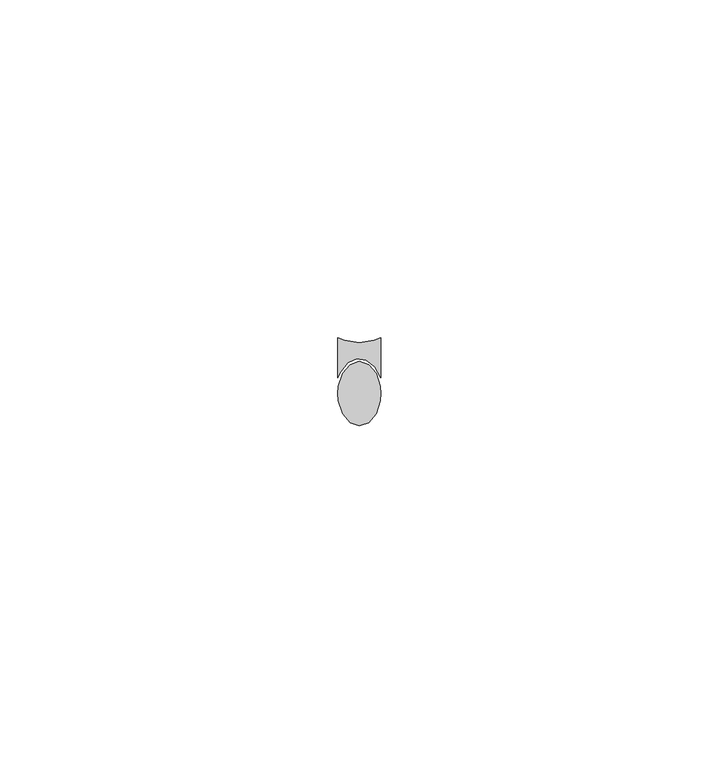
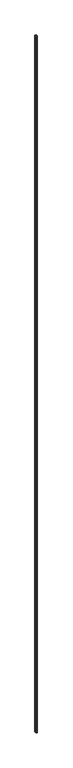
"""IFC4 building model written with IfcOpenShell, lengths in millimetres: proxy geometry, Generic Models 11:Generic Models 1:306267:Generic Models 1:306267 : Generic Models 11:Generic Models 1:306267:300405:Generic Models 1:306267:Generic Models 1:306267 : Generic Models 11:Generic Models 1:306267:300405 : Generic Models 11:Generic Models 1:306267:Generic Models 1:306267 : Generic Models 11:Generic Models 1:306267:300405:14 : Generic Models 11:Generic Models 1:306267:Generic Models 1:306267 : Generic Models 11:Generic Models 1:306267:300405:Generic Models 1:306267:Generic Models 1:306267 : Generic Models 11:Generic Models 1:306267:300405 : Generic Models 11:Generic Models 1:306267:Generic Models 1:306267 : Generic Models 11:Generic Models 1:306267:300405:300182."""

from ifc_helpers import new_model, si_unit, frame, origin, place, context, project, spatial, polyline, outline, extrude, source, transform, mapped, element, save


def generic_models_b3ea6220(model_context):
    return source(origin(), model_context, "Body", "SweptSolid", [
        extrude(outline(polyline([(593831.8341434, -568222.2903513), (593833.2117242, -568221.8187155), (593834.5893051, -568222.2903513), (593835.6940392, -568223.6118453), (593836.3071204, -568225.5214595), (593836.3867242, -568226.5812155), (593836.3071204, -568227.6409714), (593835.6940392, -568229.5505857), (593834.5893051, -568230.8720797), (593833.2117242, -568231.3437155), (593831.8341434, -568230.8720797), (593830.7294093, -568229.5505857), (593830.1163281, -568227.6409714), (593830.0367242, -568226.5812155), (593830.1163281, -568225.5214595), (593830.7294093, -568223.6118453), (593831.8341434, -568222.2903513)])), frame((0.0, 0.0, 4853.797603), z_axis=(0.0, 0.0, 1.0), x_axis=(1.0, 0.0, 0.0)), (0.0, 0.0, 1.0), 3695.7),
        extrude(outline(polyline([(593835.420961, -568218.7269044), (593836.3867242, -568218.3494958), (593836.3867242, -568224.2175879), (593835.5039354, -568222.6243712), (593834.2625513, -568221.6501662), (593832.856775, -568221.4473783), (593831.5065273, -568222.0477318), (593830.4230418, -568223.3573069), (593830.0367242, -568224.2175879), (593830.0367242, -568218.3494958), (593831.0024875, -568218.7269044), (593833.2117242, -568219.0405905), (593835.420961, -568218.7269044)])), frame((0.0, 0.0, 4853.797603), z_axis=(0.0, 0.0, 1.0), x_axis=(1.0, 0.0, 0.0)), (0.0, 0.0, 1.0), 3695.7),
    ])


if __name__ == "__main__":
    model = new_model("IFC4")
    model_context = context("Model", 3, world=origin())
    ifc_project = project(units=[si_unit("LENGTHUNIT", "METRE", prefix="MILLI")], contexts=[model_context])
    site = spatial("IfcSite", under=ifc_project)
    building = spatial("IfcBuilding", under=site)
    placement = place(None, origin())
    generic_models_shape = generic_models_b3ea6220(model_context)
    element("IfcBuildingElementProxy", 1, Name="Generic Models 11:Generic Models 1:306267:Generic Models 1:306267 : Generic Models 11:Generic Models 1:306267:300405:Generic Models 1:306267:Generic Models 1:306267 : Generic Models 11:Generic Models 1:306267:300405 : Generic Models 11:Generic Models 1:306267:Generic Models 1:306267 : Generic Models 11:Generic Models 1:306267:300405:14 : Generic Models 11:Generic Models 1:306267:Generic Models 1:306267 : Generic Models 11:Generic Models 1:306267:300405:Generic Models 1:306267:Generic Models 1:306267 : Generic Models 11:Generic Models 1:306267:300405 : Generic Models 11:Generic Models 1:306267:Generic Models 1:306267 : Generic Models 11:Generic Models 1:306267:300405:300182", ObjectType="Generic Models 11:Generic Models 1:306267:Generic Models 1:306267 : Generic Models 11:Generic Models 1:306267:300405:Generic Models 1:306267:Generic Models 1:306267 : Generic Models 11:Generic Models 1:306267:300405 : Generic Models 11:Generic Models 1:306267:Generic Models 1:306267 : Generic Models 11:Generic Models 1:306267:300405:14 : Generic Models 11:Generic Models 1:306267:Generic Models 1:306267 : Generic Models 11:Generic Models 1:306267:300405:Generic Models 1:306267:Generic Models 1:306267 : Generic Models 11:Generic Models 1:306267:300405 : Generic Models 11:Generic Models 1:306267:Generic Models 1:306267 : Generic Models 11:Generic Models 1:306267:300405:300182", at=placement, inside=building, context=model_context, shape_type="MappedRepresentation", body=[
        mapped(generic_models_shape, transform((0.0, 0.0, 0.0), x_axis=(1.0, 0.0, 0.0), y_axis=(0.0, 1.0, 0.0), z_axis=(0.0, 0.0, 1.0))),
    ])
    save(model, "model.ifc")

# Revit data of these elements
# Type "Generic Models 11:Generic Models 1:306267:Generic Models 1:306267 : Generic Models 11:Generic Models 1:306267:300405:Generic Models 1:306267:Generic Models 1:306267 : Generic Models 11:Generic Models 1:306267:300405 : Generic Models 11:Generic Models 1:306267:Generic Models 1:306267 : Generic Models 11:Generic Models 1:306267:300405:14 : Generic Models 11:Generic Models 1:306267:Generic Models 1:306267 : Generic Models 11:Generic Models 1:306267:300405:Generic Models 1:306267:Generic Models 1:306267 : Generic Models 11:Generic Models 1:306267:300405 : Generic Models 11:Generic Models 1:306267:Generic Models 1:306267 : Generic Models 11:Generic Models 1:306267:300405:300182"
#   NameOverride = "Generic Models 11:Generic Models 1:306267:Generic Models 1:306267 : Generic Models 11:Generic Models 1:306267:300405:Generic Models 1:306267:Generic Models 1:306267 : Generic Models 11:Generic Models 1:306267:300405 : Generic Models 11:Generic Models 1:306267:Generic Models 1:306267 : Generic Models 11:Generic Models 1:306267:300405:300182"
#   ObjectTypeOverride = "Generic Models 1:306267:Generic Models 1:306267 : Generic Models 11:Generic Models 1:306267:300405 : Generic Models 11:Generic Models 1:306267:Generic Models 1:306267 : Generic Models 11:Generic Models 1:306267:300405"
#   Reference = "Generic Models 1"
#   Tag = "300182"
# Element 1 (IfcBuildingElementProxy, "Generic Models 11:Generic Models 1:306267:Generic Models 1:306267 : Generic Models 11:Generic Models 1:306267:300405:Generic Models 1:306267:Generic Models 1:306267 : Generic Models 11:Generic Models 1:306267:300405 : Generic Models 11:Generic Models 1:306267:Generic Models 1:306267 : Generic Models 11:Generic Models 1:306267:300405:14 : Generic Models 11:Generic Models 1:306267:Generic Models 1:306267 : Generic Models 11:Generic Models 1:306267:300405:Generic Models 1:306267:Generic Models 1:306267 : Generic Models 11:Generic Models 1:306267:300405 : Generic Models 11:Generic Models 1:306267:Generic Models 1:306267 : Generic Models 11:Generic Models 1:306267:300405:300182")
#   Materials on its faces: "SEALANT & BACKER ROD"
# Materials
#   "SEALANT & BACKER ROD": class "Unassigned", colour RGB 120 120 120, transparency 0, Cost = 0
